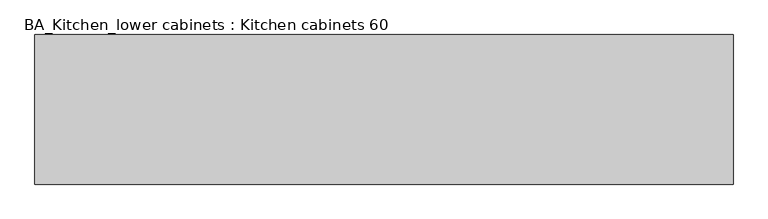
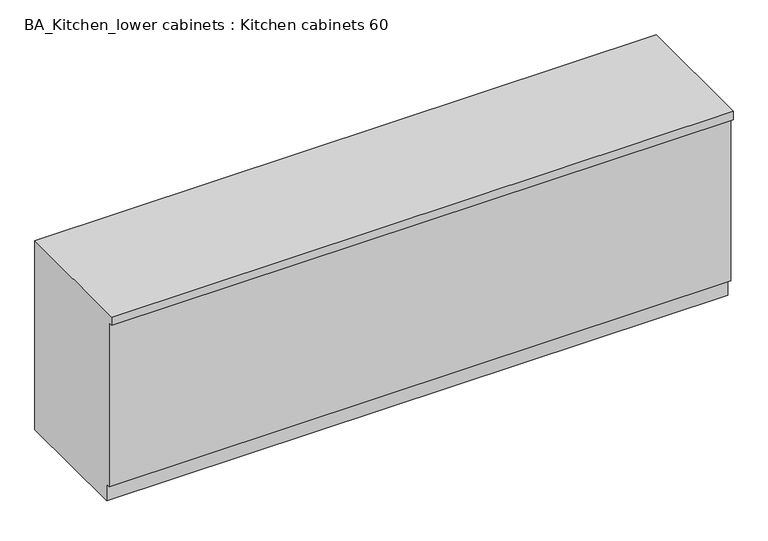
"""IFC4 building model written with IfcOpenShell, lengths in millimetres: furniture geometry, BA_Kitchen_lower cabinets : Kitchen cabinets 60."""

from ifc_helpers import new_model, si_unit, frame, origin, place, context, project, spatial, polyline, outline, extrude, source, transform, mapped, element, save


def ba_kitchen_lower_cabinets_kitchen_cabinets_60_98475e24(model_context):
    return source(origin(), model_context, "Body", "SweptSolid", [
        extrude(outline(polyline([(-600.0, 900.0), (0.0, 900.0), (0.0, 0.0), (-560.0, 0.0), (-560.0, 80.0), (-580.0, 80.0), (-580.0, 860.0), (-600.0, 860.0), (-600.0, 900.0)])), frame((0.0, 0.0, 0.0), z_axis=(1.0, 0.0, 0.0), x_axis=(0.0, 1.0, 0.0)), (0.0, 0.0, 1.0), 2800.0),
    ])


if __name__ == "__main__":
    model = new_model("IFC4")
    model_context = context("Model", 3, world=origin())
    ifc_project = project(units=[si_unit("LENGTHUNIT", "METRE", prefix="MILLI")], contexts=[model_context])
    site = spatial("IfcSite", under=ifc_project)
    building = spatial("IfcBuilding", under=site)
    placement = place(None, origin())
    ba_kitchen_lower_cabinets_kitchen_cabinets_60_shape = ba_kitchen_lower_cabinets_kitchen_cabinets_60_98475e24(model_context)
    element("IfcFurniture", 1, ObjectType="BA_Kitchen_lower cabinets : Kitchen cabinets 60", at=placement, inside=building, context=model_context, shape_type="MappedRepresentation", body=[
        mapped(ba_kitchen_lower_cabinets_kitchen_cabinets_60_shape, transform((0.0, 0.0, 0.0), x_axis=(1.0, 0.0, 0.0), y_axis=(0.0, 1.0, 0.0), z_axis=(0.0, 0.0, 1.0))),
    ])
    save(model, "model.ifc")

# Revit data of these elements
# Type "BA_Kitchen_lower cabinets : Kitchen cabinets 60"
#   built-in parameter 1001306 [instance default] = 4.85564 (stored number, unit not read)
#   Height [instance default] = 900 mm
#   Depth = 600 mm
#   Default Elevation = 0
# Element 1 (IfcFurniture, "BA_Kitchen_lower cabinets : Kitchen cabinets 60")
#   built-in parameter 1001306 = 9.18635 (stored number, unit not read)
#   Materials on its faces: "Default"
# Materials
#   "Default": class "Generic", colour RGB 255 255 255, transparency 0, Cost = 0
